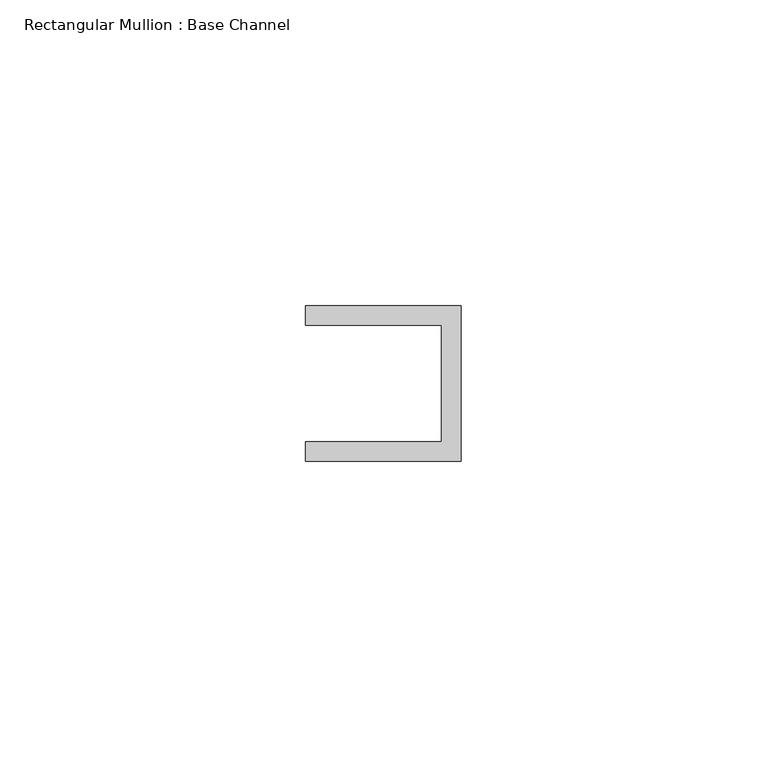
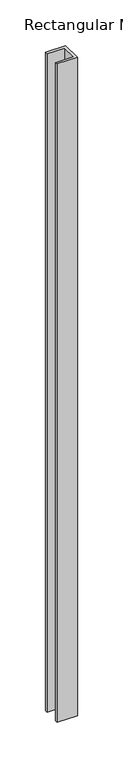
"""IFC4 building model written with IfcOpenShell, lengths in millimetres: member geometry, Rectangular Mullion : Base Channel."""

import ifcopenshell
import ifcopenshell.guid

model = None  # the IFC model being written
_history = None  # IfcOwnerHistory: only IFC2X3 demands one
_inside = {}  # id of a spatial element -> (the spatial element, [elements in it])
_under = {}  # id of a project, library or spatial element -> (it, [spatial elements below it])
_declared = {}  # id of a project -> (the project, [libraries it declares])
_typed = {}  # id of a type object -> (the type object, [elements of that type])
_made_of = {}  # id of a material, layer set ... -> (it, [elements and type objects made of it])


def new_model(schema):
    """Start an empty IFC model of exactly this schema.

    Asked for "IFC4X3", IfcOpenShell would pick the latest addendum, in which some entities
    have other attributes; the version numbers below select the first issue.
    IFC2X3 requires an IfcOwnerHistory on every rooted entity: one is made here for all.
    """
    global model, _history
    if schema == "IFC4X3":
        model = ifcopenshell.file(schema_version=(4, 3, 0, 0))
    else:
        model = ifcopenshell.file(schema=schema)
    _inside.clear()
    _under.clear()
    _declared.clear()
    _typed.clear()
    _made_of.clear()
    _history = None
    if model.schema == "IFC2X3":
        org = make("IfcOrganization", Name="unknown")
        user = make(
            "IfcPersonAndOrganization",
            ThePerson=make("IfcPerson", FamilyName="unknown"),
            TheOrganization=org,
        )
        app = make(
            "IfcApplication",
            ApplicationDeveloper=org,
            Version="unknown",
            ApplicationFullName="unknown",
            ApplicationIdentifier="unknown",
        )
        _history = make(
            "IfcOwnerHistory",
            OwningUser=user,
            OwningApplication=app,
            ChangeAction="ADDED",
            CreationDate=0,
        )
    return model


def make(cls, **values):
    """One entity of the class cls with the attributes given. An attribute that is None is left unset."""
    return model.create_entity(
        cls, **{name: value for name, value in values.items() if value is not None}
    )


def rooted(cls, **values):
    """An entity with a GlobalId (a new one), such as an element, a storey or a relation."""
    return make(cls, GlobalId=ifcopenshell.guid.new(), OwnerHistory=_history, **values)


def si_unit(unit_type, name, prefix=None):
    """IfcSIUnit, for example si_unit("LENGTHUNIT", "METRE", prefix="MILLI")."""
    return make("IfcSIUnit", UnitType=unit_type, Prefix=prefix, Name=name)


def assignment(units):
    """IfcUnitAssignment: the units of a project."""
    return None if units is None else make("IfcUnitAssignment", Units=units)


def point(xyz):
    """IfcCartesianPoint."""
    return None if xyz is None else make("IfcCartesianPoint", Coordinates=xyz)


def direction(xyz):
    """IfcDirection."""
    return None if xyz is None else make("IfcDirection", DirectionRatios=xyz)


def frame(location, z_axis=None, x_axis=None):
    """IfcAxis2Placement3D, a coordinate frame: its origin and axes. An axis left out is left unset."""
    return make(
        "IfcAxis2Placement3D",
        Location=point(location),
        Axis=direction(z_axis),
        RefDirection=direction(x_axis),
    )


def origin():
    """The frame at (0, 0, 0) with its axes left unset."""
    return frame((0.0, 0.0, 0.0))


def place(relative_to, where):
    """IfcLocalPlacement: puts the frame where relative to a parent placement (None: the world)."""
    return make(
        "IfcLocalPlacement", PlacementRelTo=relative_to, RelativePlacement=where
    )


def context(
    kind, dimensions, precision=None, world=None, true_north=None, identifier=None
):
    """IfcGeometricRepresentationContext, for example the 3D "Model" context."""
    return make(
        "IfcGeometricRepresentationContext",
        ContextIdentifier=identifier,
        ContextType=kind,
        CoordinateSpaceDimension=dimensions,
        Precision=precision,
        WorldCoordinateSystem=world,
        TrueNorth=true_north,
    )


def project(units=None, contexts=None):
    """IfcProject with its units and contexts."""
    return rooted(
        "IfcProject",
        Name="project",
        RepresentationContexts=contexts,
        UnitsInContext=assignment(units),
    )


def spatial(cls, under=None, at=None, **own):
    """A site, building, storey or space (cls), placed at a placement, below another one or the project."""
    s = rooted(cls, ObjectPlacement=at, **own)
    if under is not None:
        _under.setdefault(under.id(), (under, []))[1].append(s)
    return s


def polyline(points):
    """IfcPolyline through the points."""
    return make("IfcPolyline", Points=[point(p) for p in points])


def outline(outer, holes=None, kind="AREA"):
    """IfcArbitraryClosedProfileDef: a profile drawn as a closed curve; with holes, ...WithVoids."""
    if holes is None:
        return make("IfcArbitraryClosedProfileDef", ProfileType=kind, OuterCurve=outer)
    return make(
        "IfcArbitraryProfileDefWithVoids",
        ProfileType=kind,
        OuterCurve=outer,
        InnerCurves=holes,
    )


def extrude(swept, where, along, depth):
    """IfcExtrudedAreaSolid: the profile swept, set in the frame where, extruded along a direction by depth."""
    return make(
        "IfcExtrudedAreaSolid",
        SweptArea=swept,
        Position=where,
        ExtrudedDirection=direction(along),
        Depth=depth,
    )


def shape(context_of_items, identifier, shape_type, items):
    """IfcShapeRepresentation: the items that make up one representation, for example the "Body"."""
    return make(
        "IfcShapeRepresentation",
        ContextOfItems=context_of_items,
        RepresentationIdentifier=identifier,
        RepresentationType=shape_type,
        Items=items,
    )


def source(mapping_origin, context_of_items, identifier, shape_type, items):
    """IfcRepresentationMap: a shape defined once, which mapped items show again and again."""
    return make(
        "IfcRepresentationMap",
        MappingOrigin=mapping_origin,
        MappedRepresentation=shape(context_of_items, identifier, shape_type, items),
    )


def transform(
    local_origin,
    x_axis=None,
    y_axis=None,
    z_axis=None,
    scale=None,
    scale2=None,
    scale3=None,
    uniform=True,
):
    """IfcCartesianTransformationOperator3D, or its non-uniform kind. x_axis, y_axis, z_axis: its Axis1, 2, 3."""
    if uniform:
        return make(
            "IfcCartesianTransformationOperator3D",
            Axis1=direction(x_axis),
            Axis2=direction(y_axis),
            LocalOrigin=point(local_origin),
            Scale=scale,
            Axis3=direction(z_axis),
        )
    return make(
        "IfcCartesianTransformationOperator3DnonUniform",
        Axis1=direction(x_axis),
        Axis2=direction(y_axis),
        LocalOrigin=point(local_origin),
        Scale=scale,
        Axis3=direction(z_axis),
        Scale2=scale2,
        Scale3=scale3,
    )


def mapped(mapping_source, mapping_target):
    """IfcMappedItem: shows the shape of a source again, moved by a transform."""
    return make(
        "IfcMappedItem", MappingSource=mapping_source, MappingTarget=mapping_target
    )


def made_of(thing, what):
    """Note that an element or type object is made of a material, layer set ...; save() writes the relation."""
    if what is not None:
        _made_of.setdefault(what.id(), (what, []))[1].append(thing)
    return thing


def element(
    cls,
    number,
    at=None,
    inside=None,
    cuts=None,
    type_object=None,
    material=None,
    context=None,
    identifier="Body",
    shape_type=None,
    held_by="IfcProductDefinitionShape",
    body=None,
    shapes=None,
    **own,
):
    """One element of the class cls, such as IfcWall. Its Tag is "e" and its number.

    at: its placement. inside: the storey or other place that contains it. cuts: it is an
    opening in that element (IfcRelVoidsElement). A single representation is given by context,
    identifier, shape_type and body (its items); several are given by shapes. held_by: the class
    of the entity that holds the representations. save() writes the other relations.
    """
    e = rooted(cls, Tag="e%d" % number, ObjectPlacement=at, **own)
    if body is not None:
        shapes = [shape(context, identifier, shape_type, body)]
    if shapes is not None:
        e.Representation = make(held_by, Representations=shapes)
    if inside is not None:
        _inside.setdefault(inside.id(), (inside, []))[1].append(e)
    if cuts is not None:
        rooted(
            "IfcRelVoidsElement", RelatingBuildingElement=cuts, RelatedOpeningElement=e
        )
    if type_object is not None:
        _typed.setdefault(type_object.id(), (type_object, []))[1].append(e)
    return made_of(e, material)


def aggregate(whole, parts):
    """IfcRelAggregates: a whole, such as a stair, and the parts it consists of."""
    return rooted("IfcRelAggregates", RelatingObject=whole, RelatedObjects=parts)


def save(model, path):
    """Write the relations noted so far, then the file.

    IfcRelAggregates (storeys below a building ...), IfcRelContainedInSpatialStructure (elements
    in a storey), IfcRelDefinesByType, IfcRelAssociatesMaterial and IfcRelDeclares: one each for
    every whole, place, type object, material and project.
    """
    for whole, parts in _under.values():
        aggregate(whole, parts)
    for where, things in _inside.values():
        rooted(
            "IfcRelContainedInSpatialStructure",
            RelatedElements=things,
            RelatingStructure=where,
        )
    for kind, things in _typed.values():
        rooted("IfcRelDefinesByType", RelatedObjects=things, RelatingType=kind)
    for what, things in _made_of.values():
        rooted("IfcRelAssociatesMaterial", RelatedObjects=things, RelatingMaterial=what)
    for by, libraries in _declared.values():
        rooted("IfcRelDeclares", RelatingContext=by, RelatedDefinitions=libraries)
    model.write(path)


def rectangular_mullion_base_channel_9e3e4347(model_context):
    return source(origin(), model_context, "Body", "SweptSolid", [
        extrude(outline(polyline([(0.0, -12.7), (-25.4, -12.7), (-25.4, -9.525), (-3.175, -9.525), (-3.175, 9.525), (-25.4, 9.525), (-25.4, 12.7), (0.0, 12.7), (0.0, -12.7)])), frame((0.0, 0.0, -877.8332389), z_axis=(0.0, 0.0, 1.0), x_axis=(1.0, 0.0, 0.0)), (0.0, 0.0, 1.0), 877.8332389),
    ])


if __name__ == "__main__":
    model = new_model("IFC4")
    model_context = context("Model", 3, world=origin())
    ifc_project = project(units=[si_unit("LENGTHUNIT", "METRE", prefix="MILLI")], contexts=[model_context])
    site = spatial("IfcSite", under=ifc_project)
    building = spatial("IfcBuilding", under=site)
    placement = place(None, origin())
    rectangular_mullion_base_channel_shape = rectangular_mullion_base_channel_9e3e4347(model_context)
    element("IfcMember", 1, ObjectType="Rectangular Mullion : Base Channel", at=placement, inside=building, context=model_context, shape_type="MappedRepresentation", body=[
        mapped(rectangular_mullion_base_channel_shape, transform((0.0, 0.0, 0.0), x_axis=(1.0, 0.0, 0.0), y_axis=(0.0, 1.0, 0.0), z_axis=(0.0, 0.0, 1.0))),
    ])
    save(model, "model.ifc")

# Revit data of these elements
# Type "Rectangular Mullion : Base Channel"
#   built-in parameter 1007322 = 0.0833333 (stored number, unit not read)
#   built-in parameter 1007321 = 0.0416667 (stored number, unit not read)
#   built-in parameter 1007320 = -0.03125 (stored number, unit not read)
# Element 1 (IfcMember, "Rectangular Mullion : Base Channel")
#   Materials on its faces: "ALUM"
# Materials
#   "ALUM": class "Generic", colour RGB 157 157 157, transparency 0, Cost = 0
